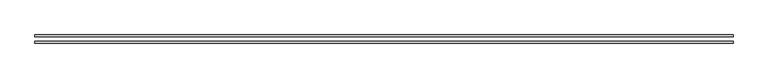
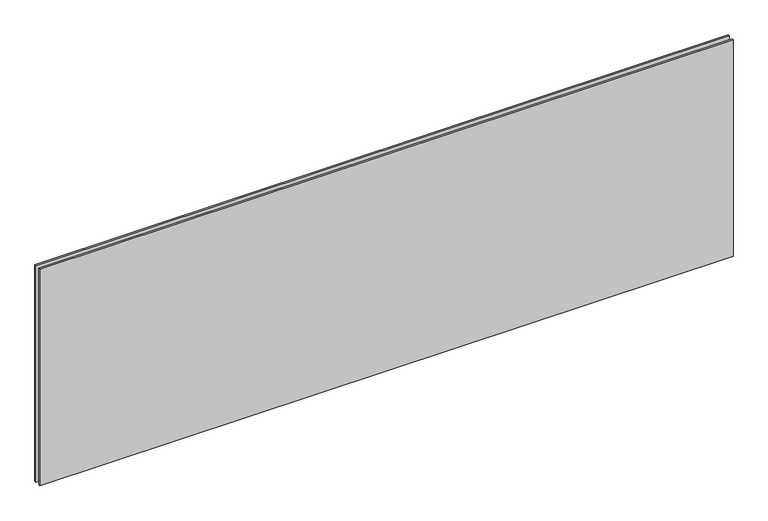
"""IFC4 building model written with IfcOpenShell, lengths in millimetres: proxy geometry, Window glass002 2265 : Window glass002 2265."""

from ifc_helpers import new_model, si_unit, frame, origin, place, context, project, spatial, polyline, outline, extrude, source, transform, mapped, element, save


def generic_models_935587b2(model_context):
    return source(origin(), model_context, "Body", "SweptSolid", [
        extrude(outline(polyline([(3694.2883192, 10421.8248386), (3694.2883192, 10426.5873386), (5694.2883192, 10426.5873386), (5694.2883192, 10421.8248386), (3694.2883192, 10421.8248386)])), frame((0.0, 0.0, 42171.7417214), z_axis=(0.0, 0.0, 1.0), x_axis=(1.0, 0.0, 0.0)), (0.0, 0.0, 1.0), 660.4),
        extrude(outline(polyline([(3694.2883192, 10440.3668386), (3694.2883192, 10445.1293386), (5694.2883192, 10445.1293386), (5694.2883192, 10440.3668386), (3694.2883192, 10440.3668386)])), frame((0.0, 0.0, 42171.7417214), z_axis=(0.0, 0.0, 1.0), x_axis=(1.0, 0.0, 0.0)), (0.0, 0.0, 1.0), 660.4),
    ])


if __name__ == "__main__":
    model = new_model("IFC4")
    model_context = context("Model", 3, world=origin())
    ifc_project = project(units=[si_unit("LENGTHUNIT", "METRE", prefix="MILLI")], contexts=[model_context])
    site = spatial("IfcSite", under=ifc_project)
    building = spatial("IfcBuilding", under=site)
    placement = place(None, origin())
    generic_models_shape = generic_models_935587b2(model_context)
    element("IfcBuildingElementProxy", 1, Name="Window glass002 2265 : Window glass002 2265", ObjectType="Window glass002 2265 : Window glass002 2265", at=placement, inside=building, context=model_context, shape_type="MappedRepresentation", body=[
        mapped(generic_models_shape, transform((0.0, 0.0, 0.0), x_axis=(1.0, 0.0, 0.0), y_axis=(0.0, 1.0, 0.0), z_axis=(0.0, 0.0, 1.0))),
    ])
    save(model, "model.ifc")

# Revit data of these elements
# Type "Window glass002 2265 : Window glass002 2265"
#   NameOverride = "Window glass002"
# Element 1 (IfcBuildingElementProxy, "Window glass002 2265 : Window glass002 2265")
#   Materials on its faces: "1\"  INSULATED GLAZING"
# Materials
#   "1\"  INSULATED GLAZING": class "Unassigned", colour RGB 146 199 212, transparency 0, Cost = 0
